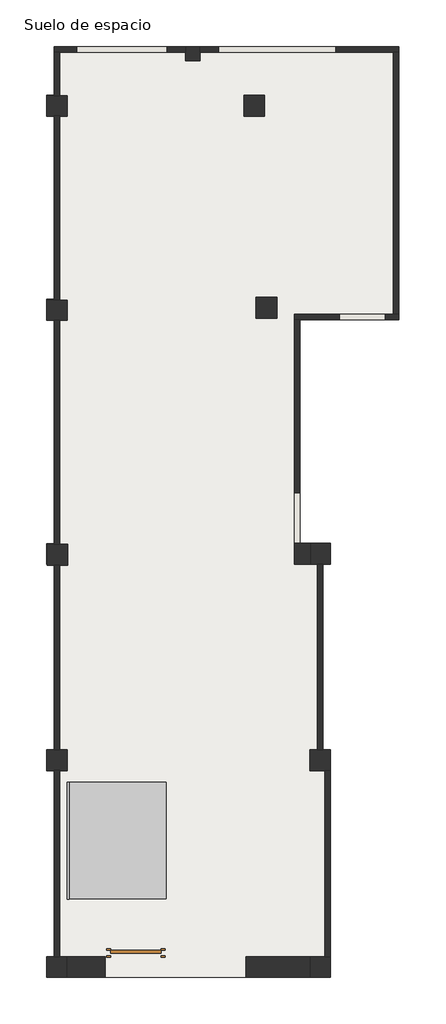
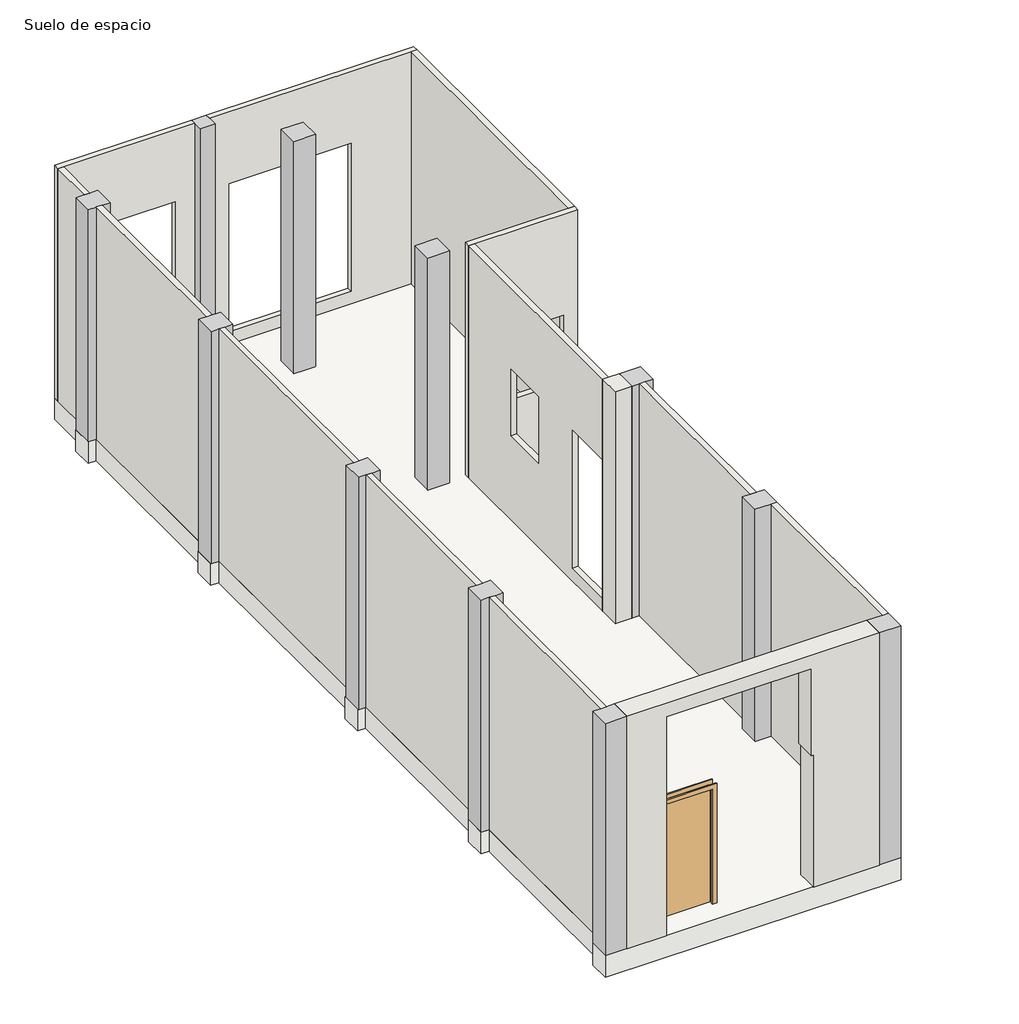
# One storey: 14 walls, 11 columns, 1 door, 1 railing, 1 ramp, 1 slab.
# Revit data of these elements (continued)
# Element 29 (IfcWall, "Generic - 380mm Masonry") (continued)
#   Base Offset = 0.0 cm
#   Unconnected Height = 430.0 cm
#   wall height = 430.0 cm
#   Phase Created = Existing
#   Base Constraint = Suelo de espacio
#   Materials on its faces: "Concrete, Cast-in-Place gray"
# Materials
#   "Door - Panel": class "Wood", colour RGB 114 82 51, transparency 0
#   "Door - Frame": class "Miscellaneous", colour RGB 153 76 43, transparency 0
#   "Concrete, Cast-in-Place gray": class "Concrete", colour RGB 115 116 108, transparency 0, Description = "Cast-in-place concrete", Cost = 0
#   "Default Roof": class "Miscellaneous", colour RGB 80 80 80, transparency 0
